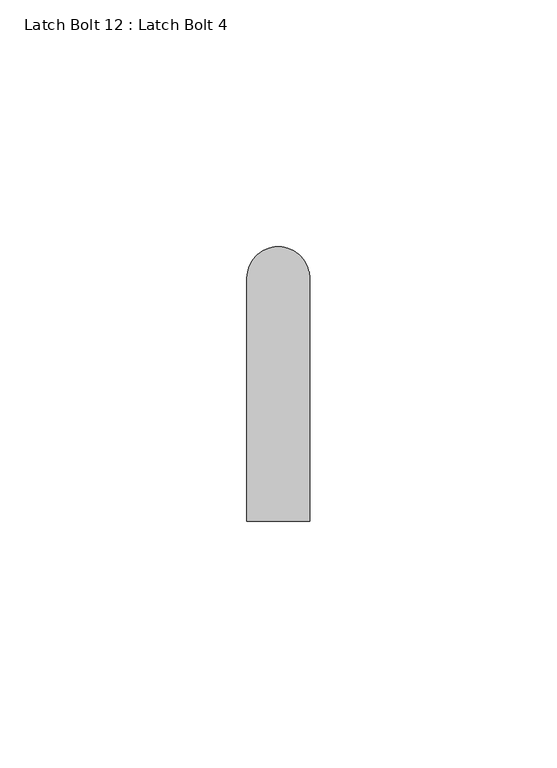
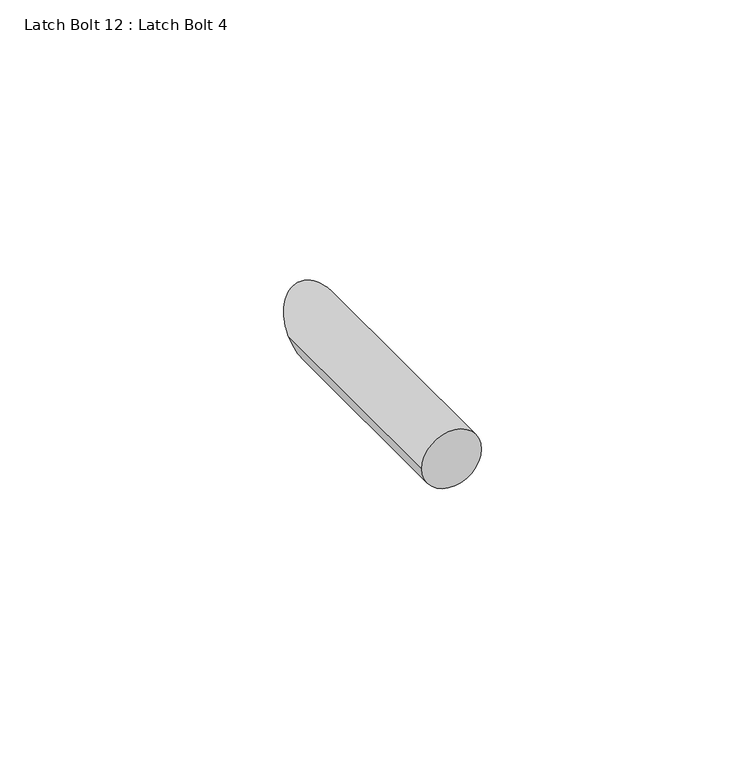
"""IFC4 building model written with IfcOpenShell, lengths in millimetres: proxy geometry, Latch Bolt 12 : Latch Bolt 4."""

import ifcopenshell
import ifcopenshell.guid

model = None  # the IFC model being written
_history = None  # IfcOwnerHistory: only IFC2X3 demands one
_inside = {}  # id of a spatial element -> (the spatial element, [elements in it])
_under = {}  # id of a project, library or spatial element -> (it, [spatial elements below it])
_declared = {}  # id of a project -> (the project, [libraries it declares])
_typed = {}  # id of a type object -> (the type object, [elements of that type])
_made_of = {}  # id of a material, layer set ... -> (it, [elements and type objects made of it])


def new_model(schema):
    """Start an empty IFC model of exactly this schema.

    Asked for "IFC4X3", IfcOpenShell would pick the latest addendum, in which some entities
    have other attributes; the version numbers below select the first issue.
    IFC2X3 requires an IfcOwnerHistory on every rooted entity: one is made here for all.
    """
    global model, _history
    if schema == "IFC4X3":
        model = ifcopenshell.file(schema_version=(4, 3, 0, 0))
    else:
        model = ifcopenshell.file(schema=schema)
    _inside.clear()
    _under.clear()
    _declared.clear()
    _typed.clear()
    _made_of.clear()
    _history = None
    if model.schema == "IFC2X3":
        org = make("IfcOrganization", Name="unknown")
        user = make(
            "IfcPersonAndOrganization",
            ThePerson=make("IfcPerson", FamilyName="unknown"),
            TheOrganization=org,
        )
        app = make(
            "IfcApplication",
            ApplicationDeveloper=org,
            Version="unknown",
            ApplicationFullName="unknown",
            ApplicationIdentifier="unknown",
        )
        _history = make(
            "IfcOwnerHistory",
            OwningUser=user,
            OwningApplication=app,
            ChangeAction="ADDED",
            CreationDate=0,
        )
    return model


def make(cls, **values):
    """One entity of the class cls with the attributes given. An attribute that is None is left unset."""
    return model.create_entity(
        cls, **{name: value for name, value in values.items() if value is not None}
    )


def rooted(cls, **values):
    """An entity with a GlobalId (a new one), such as an element, a storey or a relation."""
    return make(cls, GlobalId=ifcopenshell.guid.new(), OwnerHistory=_history, **values)


def si_unit(unit_type, name, prefix=None):
    """IfcSIUnit, for example si_unit("LENGTHUNIT", "METRE", prefix="MILLI")."""
    return make("IfcSIUnit", UnitType=unit_type, Prefix=prefix, Name=name)


def assignment(units):
    """IfcUnitAssignment: the units of a project."""
    return None if units is None else make("IfcUnitAssignment", Units=units)


def point(xyz):
    """IfcCartesianPoint."""
    return None if xyz is None else make("IfcCartesianPoint", Coordinates=xyz)


def direction(xyz):
    """IfcDirection."""
    return None if xyz is None else make("IfcDirection", DirectionRatios=xyz)


def frame(location, z_axis=None, x_axis=None):
    """IfcAxis2Placement3D, a coordinate frame: its origin and axes. An axis left out is left unset."""
    return make(
        "IfcAxis2Placement3D",
        Location=point(location),
        Axis=direction(z_axis),
        RefDirection=direction(x_axis),
    )


def origin():
    """The frame at (0, 0, 0) with its axes left unset."""
    return frame((0.0, 0.0, 0.0))


def place(relative_to, where):
    """IfcLocalPlacement: puts the frame where relative to a parent placement (None: the world)."""
    return make(
        "IfcLocalPlacement", PlacementRelTo=relative_to, RelativePlacement=where
    )


def context(
    kind, dimensions, precision=None, world=None, true_north=None, identifier=None
):
    """IfcGeometricRepresentationContext, for example the 3D "Model" context."""
    return make(
        "IfcGeometricRepresentationContext",
        ContextIdentifier=identifier,
        ContextType=kind,
        CoordinateSpaceDimension=dimensions,
        Precision=precision,
        WorldCoordinateSystem=world,
        TrueNorth=true_north,
    )


def project(units=None, contexts=None):
    """IfcProject with its units and contexts."""
    return rooted(
        "IfcProject",
        Name="project",
        RepresentationContexts=contexts,
        UnitsInContext=assignment(units),
    )


def spatial(cls, under=None, at=None, **own):
    """A site, building, storey or space (cls), placed at a placement, below another one or the project."""
    s = rooted(cls, ObjectPlacement=at, **own)
    if under is not None:
        _under.setdefault(under.id(), (under, []))[1].append(s)
    return s


def circle_curve(where, radius):
    """IfcCircle in the frame where."""
    return make("IfcCircle", Position=where, Radius=radius)


def ellipse_curve(where, semi_axis1, semi_axis2):
    """IfcEllipse in the frame where."""
    return make(
        "IfcEllipse", Position=where, SemiAxis1=semi_axis1, SemiAxis2=semi_axis2
    )


def shape(context_of_items, identifier, shape_type, items):
    """IfcShapeRepresentation: the items that make up one representation, for example the "Body"."""
    return make(
        "IfcShapeRepresentation",
        ContextOfItems=context_of_items,
        RepresentationIdentifier=identifier,
        RepresentationType=shape_type,
        Items=items,
    )


def source(mapping_origin, context_of_items, identifier, shape_type, items):
    """IfcRepresentationMap: a shape defined once, which mapped items show again and again."""
    return make(
        "IfcRepresentationMap",
        MappingOrigin=mapping_origin,
        MappedRepresentation=shape(context_of_items, identifier, shape_type, items),
    )


def transform(
    local_origin,
    x_axis=None,
    y_axis=None,
    z_axis=None,
    scale=None,
    scale2=None,
    scale3=None,
    uniform=True,
):
    """IfcCartesianTransformationOperator3D, or its non-uniform kind. x_axis, y_axis, z_axis: its Axis1, 2, 3."""
    if uniform:
        return make(
            "IfcCartesianTransformationOperator3D",
            Axis1=direction(x_axis),
            Axis2=direction(y_axis),
            LocalOrigin=point(local_origin),
            Scale=scale,
            Axis3=direction(z_axis),
        )
    return make(
        "IfcCartesianTransformationOperator3DnonUniform",
        Axis1=direction(x_axis),
        Axis2=direction(y_axis),
        LocalOrigin=point(local_origin),
        Scale=scale,
        Axis3=direction(z_axis),
        Scale2=scale2,
        Scale3=scale3,
    )


def mapped(mapping_source, mapping_target):
    """IfcMappedItem: shows the shape of a source again, moved by a transform."""
    return make(
        "IfcMappedItem", MappingSource=mapping_source, MappingTarget=mapping_target
    )


def made_of(thing, what):
    """Note that an element or type object is made of a material, layer set ...; save() writes the relation."""
    if what is not None:
        _made_of.setdefault(what.id(), (what, []))[1].append(thing)
    return thing


def element(
    cls,
    number,
    at=None,
    inside=None,
    cuts=None,
    type_object=None,
    material=None,
    context=None,
    identifier="Body",
    shape_type=None,
    held_by="IfcProductDefinitionShape",
    body=None,
    shapes=None,
    **own,
):
    """One element of the class cls, such as IfcWall. Its Tag is "e" and its number.

    at: its placement. inside: the storey or other place that contains it. cuts: it is an
    opening in that element (IfcRelVoidsElement). A single representation is given by context,
    identifier, shape_type and body (its items); several are given by shapes. held_by: the class
    of the entity that holds the representations. save() writes the other relations.
    """
    e = rooted(cls, Tag="e%d" % number, ObjectPlacement=at, **own)
    if body is not None:
        shapes = [shape(context, identifier, shape_type, body)]
    if shapes is not None:
        e.Representation = make(held_by, Representations=shapes)
    if inside is not None:
        _inside.setdefault(inside.id(), (inside, []))[1].append(e)
    if cuts is not None:
        rooted(
            "IfcRelVoidsElement", RelatingBuildingElement=cuts, RelatedOpeningElement=e
        )
    if type_object is not None:
        _typed.setdefault(type_object.id(), (type_object, []))[1].append(e)
    return made_of(e, material)


def aggregate(whole, parts):
    """IfcRelAggregates: a whole, such as a stair, and the parts it consists of."""
    return rooted("IfcRelAggregates", RelatingObject=whole, RelatedObjects=parts)


def save(model, path):
    """Write the relations noted so far, then the file.

    IfcRelAggregates (storeys below a building ...), IfcRelContainedInSpatialStructure (elements
    in a storey), IfcRelDefinesByType, IfcRelAssociatesMaterial and IfcRelDeclares: one each for
    every whole, place, type object, material and project.
    """
    for whole, parts in _under.values():
        aggregate(whole, parts)
    for where, things in _inside.values():
        rooted(
            "IfcRelContainedInSpatialStructure",
            RelatedElements=things,
            RelatingStructure=where,
        )
    for kind, things in _typed.values():
        rooted("IfcRelDefinesByType", RelatedObjects=things, RelatingType=kind)
    for what, things in _made_of.values():
        rooted("IfcRelAssociatesMaterial", RelatedObjects=things, RelatingMaterial=what)
    for by, libraries in _declared.values():
        rooted("IfcRelDeclares", RelatingContext=by, RelatedDefinitions=libraries)
    model.write(path)


def plane_surface(at):
    """IfcPlane: the flat surface through the origin of the frame at, square to its z axis."""
    return make("IfcPlane", Position=at)


def cylinder_surface(at, radius):
    """IfcCylindricalSurface: all points at the distance radius from the z axis of the frame at."""
    return make("IfcCylindricalSurface", Position=at, Radius=radius)


def advanced_brep(points, edges, surfaces, faces):
    """IfcAdvancedBrep: a solid bounded by faces that lie on surfaces and meet in shared edges.

    An edge is (start, end): straight between two places in points (the first is 0);
    or (start, end, curve); or (start, end, curve, False) where it runs against its curve.
    A face is (place in surfaces, loops), or (place, loops, False) where it looks against
    its surface's normal. A loop lists edges by number (the first is 1), with a minus sign
    where the edge is run from its end to its start. The first loop is the outer one.
    """
    corners = [point(p) for p in points]
    vertices = [make("IfcVertexPoint", VertexGeometry=c) for c in corners]
    made = []
    for start, end, *more in edges:
        made.append(
            make(
                "IfcEdgeCurve",
                EdgeStart=vertices[start],
                EdgeEnd=vertices[end],
                EdgeGeometry=more[0] if more else make("IfcPolyline", Points=[corners[start], corners[end]]),
                SameSense=more[1] if len(more) > 1 else True,
            )
        )
    hull = []
    for where, loops, *sense in faces:
        bounds = []
        for j, loop in enumerate(loops):
            ring = [make("IfcOrientedEdge", EdgeElement=made[abs(k) - 1], Orientation=k > 0) for k in loop]
            bounds.append(
                make(
                    "IfcFaceOuterBound" if j == 0 else "IfcFaceBound",
                    Bound=make("IfcEdgeLoop", EdgeList=ring),
                    Orientation=True,
                )
            )
        hull.append(make("IfcAdvancedFace", Bounds=bounds, FaceSurface=surfaces[where], SameSense=sense[0] if sense else True))
    return make("IfcAdvancedBrep", Outer=make("IfcClosedShell", CfsFaces=hull))


def latch_bolt_12_latch_bolt_4_94dad4aa(model_context):
    return source(origin(), model_context, "Body", "AdvancedBrep", [
        advanced_brep(
        [(587315.8935739, -532888.5610985, 292.1), (587303.1935739, -532888.5610985, 292.1), (587315.8935739, -532839.3485985, 292.1), (587303.1935739, -532839.3485985, 292.1)],
        [
            (0, 1, circle_curve(frame((587309.5435739, -532888.5610985, 292.1), z_axis=(0.0, -1.0, 0.0), x_axis=(1.0, 0.0, 0.0)), 6.35)),
            (1, 0, circle_curve(frame((587309.5435739, -532888.5610985, 292.1), z_axis=(0.0, -1.0, 0.0), x_axis=(1.0, 0.0, 0.0)), 6.35)),
            (0, 2),
            (2, 3, ellipse_curve(frame((587309.5435739, -532839.3485985, 292.1), z_axis=(0.0, -0.7071067811865497, 0.7071067811865455), x_axis=(0.0, -0.7071067811865454, -0.7071067811865497)), 8.9802561, 6.35)),
            (3, 1),
            (3, 2, ellipse_curve(frame((587309.5435739, -532839.3485985, 292.1), z_axis=(0.0, -0.7071067811865497, 0.7071067811865455), x_axis=(0.0, -0.7071067811865454, -0.7071067811865497)), 8.9802561, 6.35)),
        ],
        [
            plane_surface(frame((587315.8935739, -532888.5610985, 292.1), z_axis=(0.0, -1.0, 0.0), x_axis=(0.0, 0.0, 1.0))),
            cylinder_surface(frame((587309.5435739, -532831.4110985, 292.1), z_axis=(0.0, -1.0, 0.0), x_axis=(1.0, 0.0, 0.0)), 6.35),
            plane_surface(frame((587338.1185739, -532847.2860985, 284.1625), z_axis=(0.0, 0.7071067811865497, -0.7071067811865455), x_axis=(-1.0, 0.0, 0.0))),
        ],
        [
            (0, [[1, 2]]),
            (1, [[-1, 3, 4, 5]]),
            (1, [[-2, -5, 6, -3]]),
            (2, [[-4, -6]]),
        ],
    ),
    ])


if __name__ == "__main__":
    model = new_model("IFC4")
    model_context = context("Model", 3, world=origin())
    ifc_project = project(units=[si_unit("LENGTHUNIT", "METRE", prefix="MILLI")], contexts=[model_context])
    site = spatial("IfcSite", under=ifc_project)
    building = spatial("IfcBuilding", under=site)
    placement = place(None, origin())
    latch_bolt_12_latch_bolt_4_shape = latch_bolt_12_latch_bolt_4_94dad4aa(model_context)
    element("IfcBuildingElementProxy", 1, Name="Latch Bolt 12 : Latch Bolt 4", ObjectType="Latch Bolt 12 : Latch Bolt 4", at=placement, inside=building, context=model_context, shape_type="MappedRepresentation", body=[
        mapped(latch_bolt_12_latch_bolt_4_shape, transform((0.0, 0.0, 0.0), x_axis=(1.0, 0.0, 0.0), y_axis=(0.0, 1.0, 0.0), z_axis=(0.0, 0.0, 1.0))),
    ])
    save(model, "model.ifc")

# Revit data of these elements
# Element 1 (IfcBuildingElementProxy, "Latch Bolt 12 : Latch Bolt 4")
#   Materials on its faces: "GALV. SLIDE BOLT"
# Materials
#   "GALV. SLIDE BOLT": class "Metal", colour RGB 189 187 185, transparency 0, Description = "Carbon steel", Cost = 0
